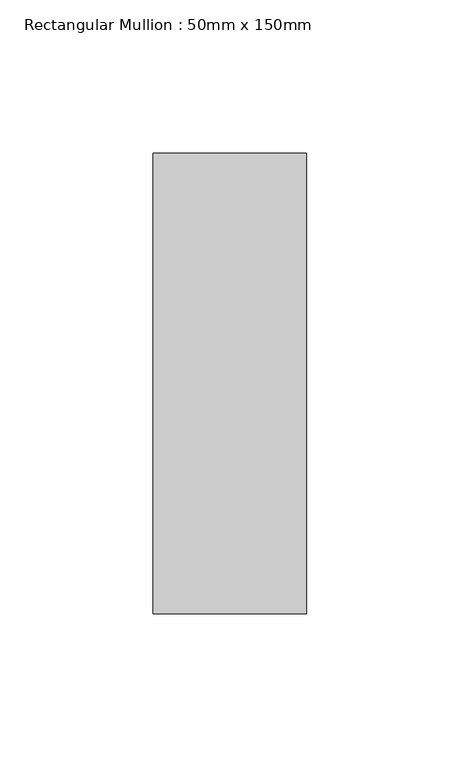
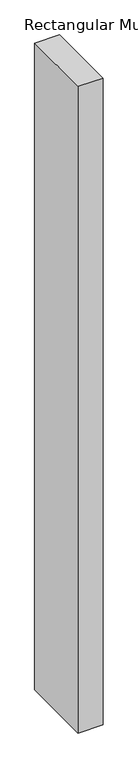
"""IFC4 building model written with IfcOpenShell, lengths in millimetres: member geometry, Rectangular Mullion : 50mm x 150mm."""

from ifc_helpers import new_model, si_unit, frame, origin, place, context, project, spatial, polyline, outline, extrude, source, transform, mapped, element, save


def rectangular_mullion_50mm_x_150mm_4fdd2d81(model_context):
    return source(origin(), model_context, "Body", "SweptSolid", [
        extrude(outline(polyline([(0.0, 75.0), (0.0, -75.0), (-50.0, -75.0), (-50.0, 75.0), (0.0, 75.0)])), frame((0.0, 0.0, -1364.9999997), z_axis=(0.0, 0.0, 1.0), x_axis=(1.0, 0.0, 0.0)), (0.0, 0.0, 1.0), 1364.9999997),
    ])


if __name__ == "__main__":
    model = new_model("IFC4")
    model_context = context("Model", 3, world=origin())
    ifc_project = project(units=[si_unit("LENGTHUNIT", "METRE", prefix="MILLI")], contexts=[model_context])
    site = spatial("IfcSite", under=ifc_project)
    building = spatial("IfcBuilding", under=site)
    placement = place(None, origin())
    rectangular_mullion_50mm_x_150mm_shape = rectangular_mullion_50mm_x_150mm_4fdd2d81(model_context)
    element("IfcMember", 1, ObjectType="Rectangular Mullion : 50mm x 150mm", at=placement, inside=building, context=model_context, shape_type="MappedRepresentation", body=[
        mapped(rectangular_mullion_50mm_x_150mm_shape, transform((0.0, 0.0, 0.0), x_axis=(1.0, 0.0, 0.0), y_axis=(0.0, 1.0, 0.0), z_axis=(0.0, 0.0, 1.0))),
    ])
    save(model, "model.ifc")

# Revit data of these elements
# Type "Rectangular Mullion : 50mm x 150mm"
#   built-in parameter 1007304 = 0.492126 (stored number, unit not read)
#   built-in parameter 1007301 = 0.082021 (stored number, unit not read)
#   built-in parameter 1007300 = 0.082021 (stored number, unit not read)
# Element 1 (IfcMember, "Rectangular Mullion : 50mm x 150mm")
#   Materials on its faces: "Aluminum"
# Materials
#   "Aluminum": class "Metal", colour RGB 244 244 244, transparency 0, Description = "Aluminum 6061", Cost = 0
